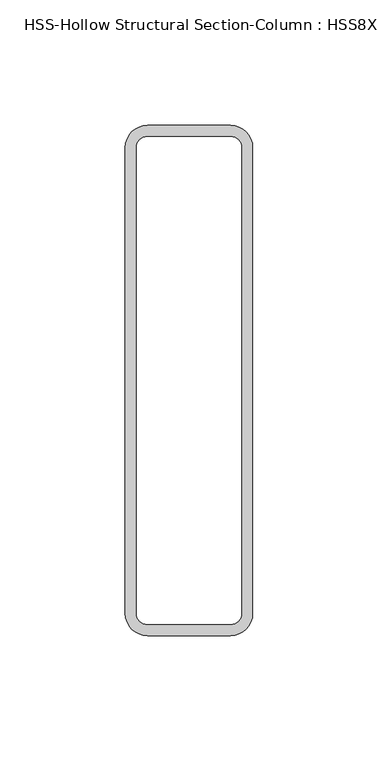
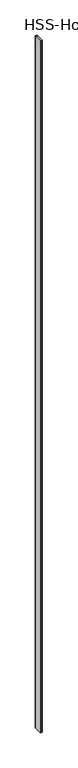
"""IFC4 building model written with IfcOpenShell, lengths in millimetres: column geometry, HSS-Hollow Structural Section-Column : HSS8X2X3/16."""

from ifc_helpers import new_model, si_unit, point, frame, frame_2d, origin, place, context, project, spatial, polyline, circle_curve, trimmed, segment, composite_curve, outline, extrude, source, transform, mapped, element, save


def hss_hollow_structural_section_column_hss8x2x3_16_37e330f9(model_context):
    return source(origin(), model_context, "Body", "SweptSolid", [
        extrude(outline(composite_curve([segment(trimmed(circle_curve(frame_2d((16.5608, 92.7608)), 8.8392), [point((16.5608, 101.6))], [point((25.4, 92.7608))], False, "CARTESIAN"), True, "CONTINUOUS"), segment(polyline([(25.4, 92.7608), (25.4, -92.7608)]), True, "CONTINUOUS"), segment(trimmed(circle_curve(frame_2d((16.5608, -92.7608)), 8.8392), [point((25.4, -92.7608))], [point((16.5608, -101.6))], False, "CARTESIAN"), True, "CONTINUOUS"), segment(polyline([(16.5608, -101.6), (-16.5608, -101.6)]), True, "CONTINUOUS"), segment(trimmed(circle_curve(frame_2d((-16.5608, -92.7608)), 8.8392), [point((-16.5608, -101.6))], [point((-25.4, -92.7608))], False, "CARTESIAN"), True, "CONTINUOUS"), segment(polyline([(-25.4, -92.7608), (-25.4, 92.7608)]), True, "CONTINUOUS"), segment(trimmed(circle_curve(frame_2d((-16.5608, 92.7608)), 8.8392), [point((-25.4, 92.7608))], [point((-16.5608, 101.6))], False, "CARTESIAN"), True, "CONTINUOUS"), segment(polyline([(-16.5608, 101.6), (16.5608, 101.6)]), True, "CONTINUOUS")], self_intersect=False), holes=[composite_curve([segment(polyline([(16.5608, 97.1804), (-16.5608, 97.1804)]), True, "CONTINUOUS"), segment(trimmed(circle_curve(frame_2d((-16.5608, 92.7608)), 4.4196), [point((-16.5608, 97.1804))], [point((-20.9804, 92.7608))], True, "CARTESIAN"), True, "CONTINUOUS"), segment(polyline([(-20.9804, 92.7608), (-20.9804, -92.7608)]), True, "CONTINUOUS"), segment(trimmed(circle_curve(frame_2d((-16.5608, -92.7608)), 4.4196), [point((-20.9804, -92.7608))], [point((-16.5608, -97.1804))], True, "CARTESIAN"), True, "CONTINUOUS"), segment(polyline([(-16.5608, -97.1804), (16.5608, -97.1804)]), True, "CONTINUOUS"), segment(trimmed(circle_curve(frame_2d((16.5608, -92.7608)), 4.4196), [point((16.5608, -97.1804))], [point((20.9804, -92.7608))], True, "CARTESIAN"), True, "CONTINUOUS"), segment(polyline([(20.9804, -92.7608), (20.9804, 92.7608)]), True, "CONTINUOUS"), segment(trimmed(circle_curve(frame_2d((16.5608, 92.7608)), 4.4196), [point((20.9804, 92.7608))], [point((16.5608, 97.1804))], True, "CARTESIAN"), True, "CONTINUOUS")], self_intersect=False)]), frame((0.0, 0.0, -3550.0), z_axis=(0.0, 0.0, 1.0), x_axis=(1.0, 0.0, 0.0)), (0.0, 0.0, 1.0), 15989.0),
    ])


if __name__ == "__main__":
    model = new_model("IFC4")
    model_context = context("Model", 3, world=origin())
    ifc_project = project(units=[si_unit("LENGTHUNIT", "METRE", prefix="MILLI")], contexts=[model_context])
    site = spatial("IfcSite", under=ifc_project)
    building = spatial("IfcBuilding", under=site)
    placement = place(None, origin())
    hss_hollow_structural_section_column_hss8x2x3_16_shape = hss_hollow_structural_section_column_hss8x2x3_16_37e330f9(model_context)
    element("IfcColumn", 1, ObjectType="HSS-Hollow Structural Section-Column : HSS8X2X3/16", at=placement, inside=building, context=model_context, shape_type="MappedRepresentation", body=[
        mapped(hss_hollow_structural_section_column_hss8x2x3_16_shape, transform((0.0, 0.0, 0.0), x_axis=(1.0, 0.0, 0.0), y_axis=(0.0, 1.0, 0.0), z_axis=(0.0, 0.0, 1.0))),
    ])
    save(model, "model.ifc")

# Revit data of these elements
# Type "HSS-Hollow Structural Section-Column : HSS8X2X3/16"
#   Assembly Code = "B10"
#   Shape = "Rect."
#   Cost = 1
#   W = 12
#   Ht = 203.2 mm
#   b = 50.8 mm
#   kr = 8.839 mm
#   t = 4.42 mm
#   A = 0.00211612 m²
#   Structural Material [instance default] = Steel ASTM A500, Grade B, Rectangular and Square
# Element 1 (IfcColumn, "HSS-Hollow Structural Section-Column : HSS8X2X3/16")
#   Structural Material = Metal - Steel 43-275
#   Materials on its faces: "Metal - Steel 43-275"
# Materials
#   "Steel ASTM A500, Grade B, Rectangular and Square": class "Metal", colour RGB 199 199 199, transparency 0, Description = "Carbon steel", Cost = 0
#   "Metal - Steel 43-275": class "Metal", colour RGB 247 247 247, transparency 0, Cost = 0
